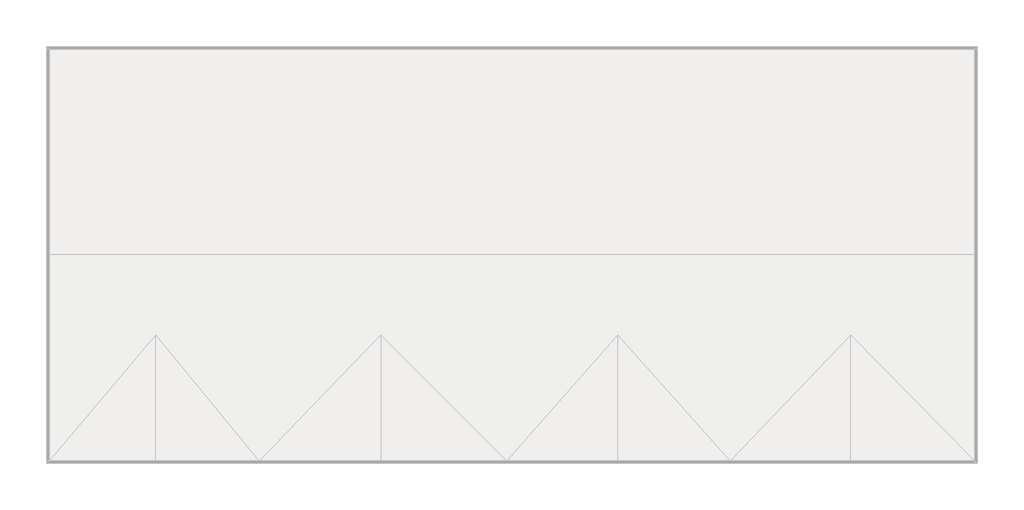
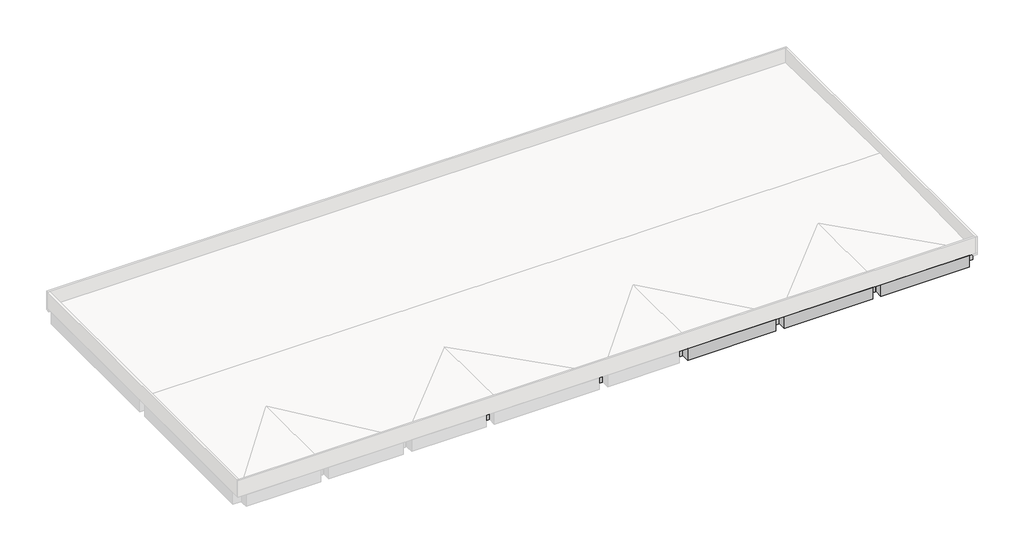
# One storey, part 2 of 2: 43 beams.
# Revit data of these elements (continued)
# Type "RC Beam_Rectangular : H_SB_AR S16_RC Beam-AG_500x900_RG3" (continued)
#   H_Rebar Ratio = 0.14
#   Width = 500 mm
#   Height = 900 mm
#   Length [instance default] = 1524 mm
#   b = 500 mm
#   h = 900 mm
#   hec_material3 [instance default] = none
#   hec_material2 [instance default] = none
#   hec_material1 [instance default] = none
#   Structural Material [instance default] = none
#   Assembly Code = ""
# Type "RC Beam_Rectangular : H_SB_AR S16_RC Beam-AG_600x900_RB2"
#   Type Comments = "AG"
#   Type Mark = "RB2"
#   중앙부 하부근 = ""
#   중앙부 상부근 = ""
#   중앙부 보조근 = ""
#   중앙부 늑근 = ""
#   외단부 하부근 = ""
#   외단부 상부근 = ""
#   외단부 보조근 = ""
#   외단부 늑근 = ""
#   부호 = ""
#   내단부 하부근 = ""
#   내단부 상부근 = ""
#   내단부 보조근 = ""
#   내단부 늑근 = ""
#   ALL 하부근 = ""
#   ALL 상부근 = ""
#   ALL 보조근 = ""
#   ALL 늑근 = ""
#   H_Rebar Ratio = 0.14
#   Width = 600 mm
#   Height = 900 mm
#   Length [instance default] = 1524 mm
#   b = 600 mm
#   h = 900 mm
#   hec_material3 [instance default] = none
#   hec_material2 [instance default] = none
#   hec_material1 [instance default] = none
#   Structural Material [instance default] = none
#   Assembly Code = ""
# Type "RC Beam_Rectangular : H_SB_AR S16_RC Beam-AG_600x900_RB3"
#   Type Comments = "AG"
#   Type Mark = "RB3"
#   중앙부 하부근 = ""
#   중앙부 상부근 = ""
#   중앙부 보조근 = ""
#   중앙부 늑근 = ""
#   외단부 하부근 = ""
#   외단부 상부근 = ""
#   외단부 보조근 = ""
#   외단부 늑근 = ""
#   부호 = ""
#   내단부 하부근 = ""
#   내단부 상부근 = ""
#   내단부 보조근 = ""
#   내단부 늑근 = ""
#   ALL 하부근 = ""
#   ALL 상부근 = ""
#   ALL 보조근 = ""
#   ALL 늑근 = ""
#   H_Rebar Ratio = 0.14
#   Width = 600 mm
#   Height = 900 mm
#   Length [instance default] = 1524 mm
#   b = 600 mm
#   h = 900 mm
#   hec_material3 [instance default] = none
#   hec_material2 [instance default] = none
#   hec_material1 [instance default] = none
#   Structural Material [instance default] = none
#   Assembly Code = ""
# Elements 1, 2, 3, 4, 5, 6, 7, 8, 9, 10, 11 (IfcBeam, "RC Beam_Rectangular : H_SB_AR S16_RC Beam-AG_600x900_RG9")
#   hec_material3 = none
#   hec_material2 = none
#   hec_material1 = none
#   Structural Material = 00_Concrete_Reinf. Conc.
#   Phase Created = New Construction
#   Materials on its faces: "00_Concrete_Reinf. Conc."
# Element 12 (IfcBeam, "RC Beam_Rectangular : H_SB_AR S16_RC Beam-AG_600x900_RG7")
#   hec_material3 = none
#   hec_material2 = none
#   hec_material1 = none
#   Structural Material = 00_Concrete_Reinf. Conc.
#   Phase Created = New Construction
#   Materials on its faces: "00_Concrete_Reinf. Conc."
# Element 13 (IfcBeam, "RC Beam_Rectangular : H_SB_AR S16_RC Beam-AG_600x900_RG8")
#   hec_material3 = none
#   hec_material2 = none
#   hec_material1 = none
#   Structural Material = 00_Concrete_Reinf. Conc.
#   Phase Created = New Construction
#   Materials on its faces: "00_Concrete_Reinf. Conc."
# Elements 14, 15, 16, 17 (IfcBeam, "RC Beam_Rectangular : H_SB_AR S16_RC Beam-AG_600x900_RG5")
#   hec_material3 = none
#   hec_material2 = none
#   hec_material1 = none
#   Structural Material = 00_Concrete_Reinf. Conc.
#   Phase Created = New Construction
#   Materials on its faces: "00_Concrete_Reinf. Conc."
# Element 18 (IfcBeam, "RC Beam_Rectangular : H_SB_AR S16_RC Beam-AG_600x900_RG5A")
#   hec_material3 = none
#   hec_material2 = none
#   hec_material1 = none
#   Structural Material = 00_Concrete_Reinf. Conc.
#   Phase Created = New Construction
#   Materials on its faces: "00_Concrete_Reinf. Conc."
# Elements 19, 20 (IfcBeam, "RC Beam_Rectangular : H_SB_AR S16_RC Beam-AG_600x900_RG4")
#   hec_material3 = none
#   hec_material2 = none
#   hec_material1 = none
#   Structural Material = 00_Concrete_Reinf. Conc.
#   Phase Created = New Construction
#   Materials on its faces: "00_Concrete_Reinf. Conc."
# Elements 21, 22 (IfcBeam, "RC Beam_Rectangular : H_SB_AR S16_RC Beam-AG_600x900_RG1A")
#   hec_material3 = none
#   hec_material2 = none
#   hec_material1 = none
#   Structural Material = 00_Concrete_Reinf. Conc.
#   Phase Created = New Construction
#   Materials on its faces: "00_Concrete_Reinf. Conc."
# Element 23 (IfcBeam, "RC Beam_Rectangular : H_SB_AR S16_RC Beam-AG_400x900_RG1")
#   hec_material3 = none
#   hec_material2 = none
#   hec_material1 = none
#   Structural Material = 00_Concrete_Reinf. Conc.
#   Phase Created = New Construction
#   Materials on its faces: "00_Concrete_Reinf. Conc."
# Elements 24, 25 (IfcBeam, "RC Beam_Rectangular : H_SB_AR S16_RC Beam-AG_400x900_RB1")
#   hec_material3 = none
#   hec_material2 = none
#   hec_material1 = none
#   Structural Material = 00_Concrete_Reinf. Conc.
#   Phase Created = New Construction
#   Materials on its faces: "00_Concrete_Reinf. Conc."
# Elements 26, 28, 30, 32 (IfcBeam, "RC Beam_Rectangular : H_SB_AR S16_RC Beam-AG_500x900_RG2")
#   hec_material3 = none
#   hec_material2 = none
#   hec_material1 = none
#   Structural Material = 00_Concrete_Reinf. Conc.
#   Phase Created = New Construction
#   Materials on its faces: "00_Concrete_Reinf. Conc."
# Elements 27, 29, 31, 33 (IfcBeam, "RC Beam_Rectangular : H_SB_AR S16_RC Beam-AG_500x900_RG3")
#   hec_material3 = none
#   hec_material2 = none
#   hec_material1 = none
#   Structural Material = 00_Concrete_Reinf. Conc.
#   Phase Created = New Construction
#   Materials on its faces: "00_Concrete_Reinf. Conc."
# Elements 34, 36, 38, 40, 42 (IfcBeam, "RC Beam_Rectangular : H_SB_AR S16_RC Beam-AG_600x900_RB2")
#   hec_material3 = none
#   hec_material2 = none
#   hec_material1 = none
#   Structural Material = 00_Concrete_Reinf. Conc.
#   Phase Created = New Construction
#   Materials on its faces: "00_Concrete_Reinf. Conc."
# Elements 35, 37, 39, 41, 43 (IfcBeam, "RC Beam_Rectangular : H_SB_AR S16_RC Beam-AG_600x900_RB3")
#   hec_material3 = none
#   hec_material2 = none
#   hec_material1 = none
#   Structural Material = 00_Concrete_Reinf. Conc.
#   Phase Created = New Construction
#   Materials on its faces: "00_Concrete_Reinf. Conc."
# Materials
#   "00_Concrete_Reinf. Conc.": class "Concrete", colour RGB 176 176 176, transparency 0, Description = "Reinf. Conc.", Cost = 0, Image = Concrete.Cast-In-Place.Flat.Polished.Grey.jpg
